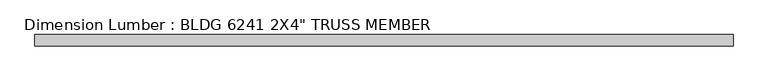
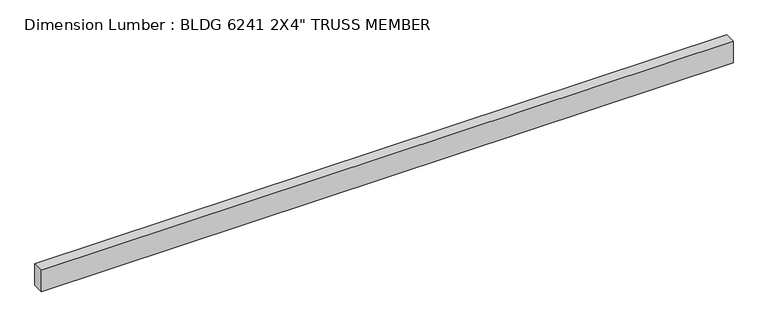
"""IFC4 building model written with IfcOpenShell, lengths in millimetres: beam geometry."""

import ifcopenshell
import ifcopenshell.guid

model = None  # the IFC model being written
_history = None  # IfcOwnerHistory: only IFC2X3 demands one
_inside = {}  # id of a spatial element -> (the spatial element, [elements in it])
_under = {}  # id of a project, library or spatial element -> (it, [spatial elements below it])
_declared = {}  # id of a project -> (the project, [libraries it declares])
_typed = {}  # id of a type object -> (the type object, [elements of that type])
_made_of = {}  # id of a material, layer set ... -> (it, [elements and type objects made of it])


def new_model(schema):
    """Start an empty IFC model of exactly this schema.

    Asked for "IFC4X3", IfcOpenShell would pick the latest addendum, in which some entities
    have other attributes; the version numbers below select the first issue.
    IFC2X3 requires an IfcOwnerHistory on every rooted entity: one is made here for all.
    """
    global model, _history
    if schema == "IFC4X3":
        model = ifcopenshell.file(schema_version=(4, 3, 0, 0))
    else:
        model = ifcopenshell.file(schema=schema)
    _inside.clear()
    _under.clear()
    _declared.clear()
    _typed.clear()
    _made_of.clear()
    _history = None
    if model.schema == "IFC2X3":
        org = make("IfcOrganization", Name="unknown")
        user = make(
            "IfcPersonAndOrganization",
            ThePerson=make("IfcPerson", FamilyName="unknown"),
            TheOrganization=org,
        )
        app = make(
            "IfcApplication",
            ApplicationDeveloper=org,
            Version="unknown",
            ApplicationFullName="unknown",
            ApplicationIdentifier="unknown",
        )
        _history = make(
            "IfcOwnerHistory",
            OwningUser=user,
            OwningApplication=app,
            ChangeAction="ADDED",
            CreationDate=0,
        )
    return model


def make(cls, **values):
    """One entity of the class cls with the attributes given. An attribute that is None is left unset."""
    return model.create_entity(
        cls, **{name: value for name, value in values.items() if value is not None}
    )


def rooted(cls, **values):
    """An entity with a GlobalId (a new one), such as an element, a storey or a relation."""
    return make(cls, GlobalId=ifcopenshell.guid.new(), OwnerHistory=_history, **values)


def si_unit(unit_type, name, prefix=None):
    """IfcSIUnit, for example si_unit("LENGTHUNIT", "METRE", prefix="MILLI")."""
    return make("IfcSIUnit", UnitType=unit_type, Prefix=prefix, Name=name)


def assignment(units):
    """IfcUnitAssignment: the units of a project."""
    return None if units is None else make("IfcUnitAssignment", Units=units)


def point(xyz):
    """IfcCartesianPoint."""
    return None if xyz is None else make("IfcCartesianPoint", Coordinates=xyz)


def direction(xyz):
    """IfcDirection."""
    return None if xyz is None else make("IfcDirection", DirectionRatios=xyz)


def frame(location, z_axis=None, x_axis=None):
    """IfcAxis2Placement3D, a coordinate frame: its origin and axes. An axis left out is left unset."""
    return make(
        "IfcAxis2Placement3D",
        Location=point(location),
        Axis=direction(z_axis),
        RefDirection=direction(x_axis),
    )


def origin():
    """The frame at (0, 0, 0) with its axes left unset."""
    return frame((0.0, 0.0, 0.0))


def place(relative_to, where):
    """IfcLocalPlacement: puts the frame where relative to a parent placement (None: the world)."""
    return make(
        "IfcLocalPlacement", PlacementRelTo=relative_to, RelativePlacement=where
    )


def context(
    kind, dimensions, precision=None, world=None, true_north=None, identifier=None
):
    """IfcGeometricRepresentationContext, for example the 3D "Model" context."""
    return make(
        "IfcGeometricRepresentationContext",
        ContextIdentifier=identifier,
        ContextType=kind,
        CoordinateSpaceDimension=dimensions,
        Precision=precision,
        WorldCoordinateSystem=world,
        TrueNorth=true_north,
    )


def project(units=None, contexts=None):
    """IfcProject with its units and contexts."""
    return rooted(
        "IfcProject",
        Name="project",
        RepresentationContexts=contexts,
        UnitsInContext=assignment(units),
    )


def spatial(cls, under=None, at=None, **own):
    """A site, building, storey or space (cls), placed at a placement, below another one or the project."""
    s = rooted(cls, ObjectPlacement=at, **own)
    if under is not None:
        _under.setdefault(under.id(), (under, []))[1].append(s)
    return s


def polyline(points):
    """IfcPolyline through the points."""
    return make("IfcPolyline", Points=[point(p) for p in points])


def outline(outer, holes=None, kind="AREA"):
    """IfcArbitraryClosedProfileDef: a profile drawn as a closed curve; with holes, ...WithVoids."""
    if holes is None:
        return make("IfcArbitraryClosedProfileDef", ProfileType=kind, OuterCurve=outer)
    return make(
        "IfcArbitraryProfileDefWithVoids",
        ProfileType=kind,
        OuterCurve=outer,
        InnerCurves=holes,
    )


def extrude(swept, where, along, depth):
    """IfcExtrudedAreaSolid: the profile swept, set in the frame where, extruded along a direction by depth."""
    return make(
        "IfcExtrudedAreaSolid",
        SweptArea=swept,
        Position=where,
        ExtrudedDirection=direction(along),
        Depth=depth,
    )


def shape(context_of_items, identifier, shape_type, items):
    """IfcShapeRepresentation: the items that make up one representation, for example the "Body"."""
    return make(
        "IfcShapeRepresentation",
        ContextOfItems=context_of_items,
        RepresentationIdentifier=identifier,
        RepresentationType=shape_type,
        Items=items,
    )


def source(mapping_origin, context_of_items, identifier, shape_type, items):
    """IfcRepresentationMap: a shape defined once, which mapped items show again and again."""
    return make(
        "IfcRepresentationMap",
        MappingOrigin=mapping_origin,
        MappedRepresentation=shape(context_of_items, identifier, shape_type, items),
    )


def transform(
    local_origin,
    x_axis=None,
    y_axis=None,
    z_axis=None,
    scale=None,
    scale2=None,
    scale3=None,
    uniform=True,
):
    """IfcCartesianTransformationOperator3D, or its non-uniform kind. x_axis, y_axis, z_axis: its Axis1, 2, 3."""
    if uniform:
        return make(
            "IfcCartesianTransformationOperator3D",
            Axis1=direction(x_axis),
            Axis2=direction(y_axis),
            LocalOrigin=point(local_origin),
            Scale=scale,
            Axis3=direction(z_axis),
        )
    return make(
        "IfcCartesianTransformationOperator3DnonUniform",
        Axis1=direction(x_axis),
        Axis2=direction(y_axis),
        LocalOrigin=point(local_origin),
        Scale=scale,
        Axis3=direction(z_axis),
        Scale2=scale2,
        Scale3=scale3,
    )


def mapped(mapping_source, mapping_target):
    """IfcMappedItem: shows the shape of a source again, moved by a transform."""
    return make(
        "IfcMappedItem", MappingSource=mapping_source, MappingTarget=mapping_target
    )


def made_of(thing, what):
    """Note that an element or type object is made of a material, layer set ...; save() writes the relation."""
    if what is not None:
        _made_of.setdefault(what.id(), (what, []))[1].append(thing)
    return thing


def element(
    cls,
    number,
    at=None,
    inside=None,
    cuts=None,
    type_object=None,
    material=None,
    context=None,
    identifier="Body",
    shape_type=None,
    held_by="IfcProductDefinitionShape",
    body=None,
    shapes=None,
    **own,
):
    """One element of the class cls, such as IfcWall. Its Tag is "e" and its number.

    at: its placement. inside: the storey or other place that contains it. cuts: it is an
    opening in that element (IfcRelVoidsElement). A single representation is given by context,
    identifier, shape_type and body (its items); several are given by shapes. held_by: the class
    of the entity that holds the representations. save() writes the other relations.
    """
    e = rooted(cls, Tag="e%d" % number, ObjectPlacement=at, **own)
    if body is not None:
        shapes = [shape(context, identifier, shape_type, body)]
    if shapes is not None:
        e.Representation = make(held_by, Representations=shapes)
    if inside is not None:
        _inside.setdefault(inside.id(), (inside, []))[1].append(e)
    if cuts is not None:
        rooted(
            "IfcRelVoidsElement", RelatingBuildingElement=cuts, RelatedOpeningElement=e
        )
    if type_object is not None:
        _typed.setdefault(type_object.id(), (type_object, []))[1].append(e)
    return made_of(e, material)


def aggregate(whole, parts):
    """IfcRelAggregates: a whole, such as a stair, and the parts it consists of."""
    return rooted("IfcRelAggregates", RelatingObject=whole, RelatedObjects=parts)


def save(model, path):
    """Write the relations noted so far, then the file.

    IfcRelAggregates (storeys below a building ...), IfcRelContainedInSpatialStructure (elements
    in a storey), IfcRelDefinesByType, IfcRelAssociatesMaterial and IfcRelDeclares: one each for
    every whole, place, type object, material and project.
    """
    for whole, parts in _under.values():
        aggregate(whole, parts)
    for where, things in _inside.values():
        rooted(
            "IfcRelContainedInSpatialStructure",
            RelatedElements=things,
            RelatingStructure=where,
        )
    for kind, things in _typed.values():
        rooted("IfcRelDefinesByType", RelatedObjects=things, RelatingType=kind)
    for what, things in _made_of.values():
        rooted("IfcRelAssociatesMaterial", RelatedObjects=things, RelatingMaterial=what)
    for by, libraries in _declared.values():
        rooted("IfcRelDeclares", RelatingContext=by, RelatedDefinitions=libraries)
    model.write(path)


def beam_e838d316(model_context):
    return source(origin(), model_context, "Body", "SweptSolid", [
        extrude(outline(polyline([(1561.1045551, 25.4), (1561.1045551, -25.4), (-1572.5300502, -25.4), (-1572.5300502, 25.4), (1561.1045551, 25.4)])), frame((0.0, 0.0, -50.8), z_axis=(0.0, 0.0, 1.0), x_axis=(1.0, 0.0, 0.0)), (0.0, 0.0, 1.0), 101.6),
    ])


if __name__ == "__main__":
    model = new_model("IFC4")
    model_context = context("Model", 3, world=origin())
    ifc_project = project(units=[si_unit("LENGTHUNIT", "METRE", prefix="MILLI")], contexts=[model_context])
    site = spatial("IfcSite", under=ifc_project)
    building = spatial("IfcBuilding", under=site)
    placement = place(None, origin())
    beam_shape = beam_e838d316(model_context)
    element("IfcBeam", 1, ObjectType="Dimension Lumber : BLDG 6241 2X4\" TRUSS MEMBER", at=placement, inside=building, context=model_context, shape_type="MappedRepresentation", body=[
        mapped(beam_shape, transform((0.0, 0.0, 0.0), x_axis=(1.0, 0.0, 0.0), y_axis=(0.0, 1.0, 0.0), z_axis=(0.0, 0.0, 1.0))),
    ])
    save(model, "model.ifc")

# Revit data of these elements
# Type "Dimension Lumber : BLDG 6241 2X4\" TRUSS MEMBER"
#   Assembly Code = "B10"
#   A = 0.273472 SF
#   Length [instance default] = 5' - 0"
#   b = 0' - 2"
#   d = 0' - 4"
#   Structural Material [instance default] = Softwood, Lumber
# Element 1 (IfcBeam, "Dimension Lumber : BLDG 6241 2X4\" TRUSS MEMBER")
#   Materials on its faces: "Softwood, Lumber"
# Materials
#   "Softwood, Lumber": class "Wood", colour RGB 223 192 134, transparency 0, Description = "Pinus Echinata", Cost = 0
